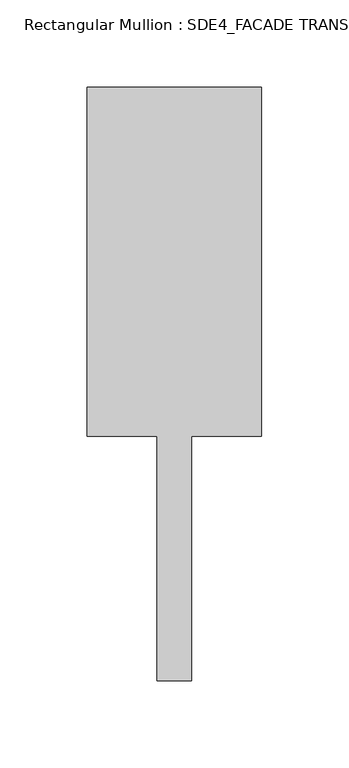
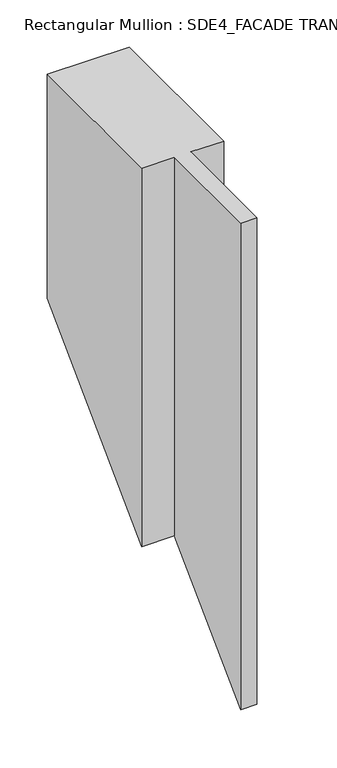
"""IFC4 building model written with IfcOpenShell, lengths in millimetres: member geometry, Rectangular Mullion : SDE4_FACADE TRANSOM TYPE 1."""

from ifc_helpers import new_model, si_unit, origin, place, context, project, spatial, faceted_brep, source, transform, mapped, element, save


def rectangular_mullion_sde4_facade_transom_type_1_c9be5fba(model_context):
    return source(origin(), model_context, "Body", "Brep", [
        faceted_brep([(50.0, 132.5, 0.0), (-50.0, 132.5, 0.0), (-50.0, -67.5, 0.0), (-10.0, -67.5, 0.0), (-10.0, -207.5, 0.0), (10.0, -207.5, 0.0), (10.0, -67.5, 0.0), (50.0, -67.5, 0.0), (50.0, 132.5, -289.0), (-50.0, 132.5, -289.0), (-50.0, -67.5, -489.0), (-10.0, -67.5, -489.0), (-10.0, -207.5, -629.0), (10.0, -207.5, -629.0), (10.0, -67.5, -489.0), (50.0, -67.5, -489.0)], [[[0, 1, 2, 3, 4, 5, 6, 7]], [[1, 0, 8, 9]], [[2, 1, 9, 10]], [[3, 2, 10, 11]], [[4, 3, 11, 12]], [[5, 4, 12, 13]], [[6, 5, 13, 14]], [[7, 6, 14, 15]], [[0, 7, 15, 8]], [[8, 15, 14, 13, 12, 11, 10, 9]]]),
    ])


if __name__ == "__main__":
    model = new_model("IFC4")
    model_context = context("Model", 3, world=origin())
    ifc_project = project(units=[si_unit("LENGTHUNIT", "METRE", prefix="MILLI")], contexts=[model_context])
    site = spatial("IfcSite", under=ifc_project)
    building = spatial("IfcBuilding", under=site)
    placement = place(None, origin())
    rectangular_mullion_sde4_facade_transom_type_1_shape = rectangular_mullion_sde4_facade_transom_type_1_c9be5fba(model_context)
    element("IfcMember", 1, ObjectType="Rectangular Mullion : SDE4_FACADE TRANSOM TYPE 1", at=placement, inside=building, context=model_context, shape_type="MappedRepresentation", body=[
        mapped(rectangular_mullion_sde4_facade_transom_type_1_shape, transform((0.0, 0.0, 0.0), x_axis=(1.0, 0.0, 0.0), y_axis=(0.0, 1.0, 0.0), z_axis=(0.0, 0.0, 1.0))),
    ])
    save(model, "model.ifc")

# Revit data of these elements
# Type "Rectangular Mullion : SDE4_FACADE TRANSOM TYPE 1"
#   built-in parameter 1007322 = 1.11549 (stored number, unit not read)
#   built-in parameter 1007321 = 0.164042 (stored number, unit not read)
#   built-in parameter 1007320 = 0.164042 (stored number, unit not read)
